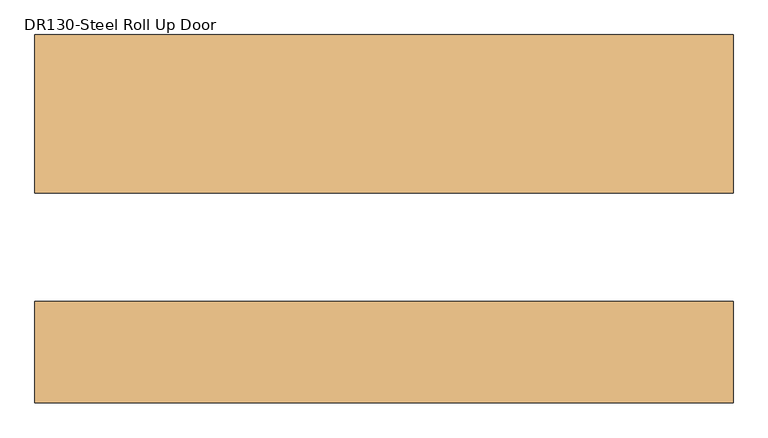
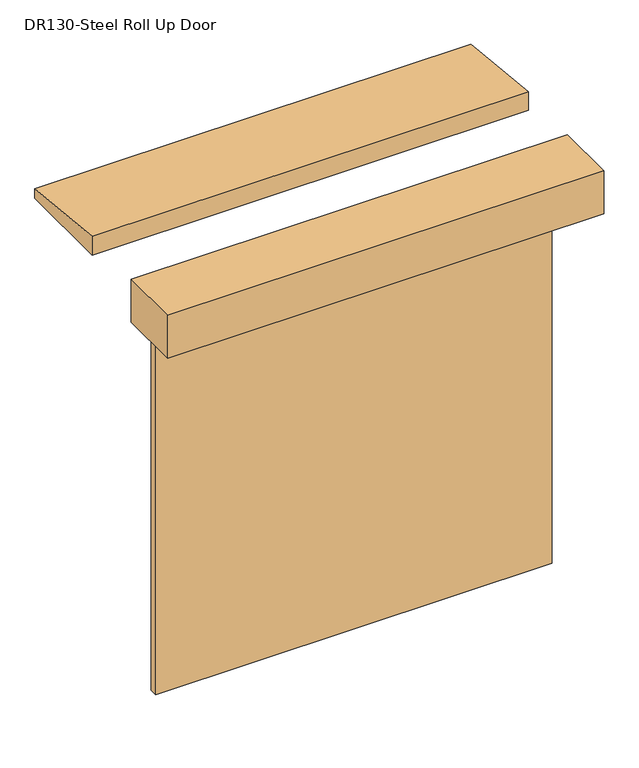
"""IFC4 building model written with IfcOpenShell, lengths in millimetres: door geometry, DR130-Steel Roll Up Door : DR131-Steel Roll Up Door-W4000xH4000mm."""

import ifcopenshell
import ifcopenshell.guid

model = None  # the IFC model being written
_history = None  # IfcOwnerHistory: only IFC2X3 demands one
_inside = {}  # id of a spatial element -> (the spatial element, [elements in it])
_under = {}  # id of a project, library or spatial element -> (it, [spatial elements below it])
_declared = {}  # id of a project -> (the project, [libraries it declares])
_typed = {}  # id of a type object -> (the type object, [elements of that type])
_made_of = {}  # id of a material, layer set ... -> (it, [elements and type objects made of it])


def new_model(schema):
    """Start an empty IFC model of exactly this schema.

    Asked for "IFC4X3", IfcOpenShell would pick the latest addendum, in which some entities
    have other attributes; the version numbers below select the first issue.
    IFC2X3 requires an IfcOwnerHistory on every rooted entity: one is made here for all.
    """
    global model, _history
    if schema == "IFC4X3":
        model = ifcopenshell.file(schema_version=(4, 3, 0, 0))
    else:
        model = ifcopenshell.file(schema=schema)
    _inside.clear()
    _under.clear()
    _declared.clear()
    _typed.clear()
    _made_of.clear()
    _history = None
    if model.schema == "IFC2X3":
        org = make("IfcOrganization", Name="unknown")
        user = make(
            "IfcPersonAndOrganization",
            ThePerson=make("IfcPerson", FamilyName="unknown"),
            TheOrganization=org,
        )
        app = make(
            "IfcApplication",
            ApplicationDeveloper=org,
            Version="unknown",
            ApplicationFullName="unknown",
            ApplicationIdentifier="unknown",
        )
        _history = make(
            "IfcOwnerHistory",
            OwningUser=user,
            OwningApplication=app,
            ChangeAction="ADDED",
            CreationDate=0,
        )
    return model


def make(cls, **values):
    """One entity of the class cls with the attributes given. An attribute that is None is left unset."""
    return model.create_entity(
        cls, **{name: value for name, value in values.items() if value is not None}
    )


def rooted(cls, **values):
    """An entity with a GlobalId (a new one), such as an element, a storey or a relation."""
    return make(cls, GlobalId=ifcopenshell.guid.new(), OwnerHistory=_history, **values)


def si_unit(unit_type, name, prefix=None):
    """IfcSIUnit, for example si_unit("LENGTHUNIT", "METRE", prefix="MILLI")."""
    return make("IfcSIUnit", UnitType=unit_type, Prefix=prefix, Name=name)


def assignment(units):
    """IfcUnitAssignment: the units of a project."""
    return None if units is None else make("IfcUnitAssignment", Units=units)


def point(xyz):
    """IfcCartesianPoint."""
    return None if xyz is None else make("IfcCartesianPoint", Coordinates=xyz)


def direction(xyz):
    """IfcDirection."""
    return None if xyz is None else make("IfcDirection", DirectionRatios=xyz)


def frame(location, z_axis=None, x_axis=None):
    """IfcAxis2Placement3D, a coordinate frame: its origin and axes. An axis left out is left unset."""
    return make(
        "IfcAxis2Placement3D",
        Location=point(location),
        Axis=direction(z_axis),
        RefDirection=direction(x_axis),
    )


def origin():
    """The frame at (0, 0, 0) with its axes left unset."""
    return frame((0.0, 0.0, 0.0))


def origin_with_axes():
    """The frame at (0, 0, 0) with the z axis (0, 0, 1) and the x axis (1, 0, 0) written out."""
    return frame((0.0, 0.0, 0.0), z_axis=(0.0, 0.0, 1.0), x_axis=(1.0, 0.0, 0.0))


def place(relative_to, where):
    """IfcLocalPlacement: puts the frame where relative to a parent placement (None: the world)."""
    return make(
        "IfcLocalPlacement", PlacementRelTo=relative_to, RelativePlacement=where
    )


def context(
    kind, dimensions, precision=None, world=None, true_north=None, identifier=None
):
    """IfcGeometricRepresentationContext, for example the 3D "Model" context."""
    return make(
        "IfcGeometricRepresentationContext",
        ContextIdentifier=identifier,
        ContextType=kind,
        CoordinateSpaceDimension=dimensions,
        Precision=precision,
        WorldCoordinateSystem=world,
        TrueNorth=true_north,
    )


def project(units=None, contexts=None):
    """IfcProject with its units and contexts."""
    return rooted(
        "IfcProject",
        Name="project",
        RepresentationContexts=contexts,
        UnitsInContext=assignment(units),
    )


def spatial(cls, under=None, at=None, **own):
    """A site, building, storey or space (cls), placed at a placement, below another one or the project."""
    s = rooted(cls, ObjectPlacement=at, **own)
    if under is not None:
        _under.setdefault(under.id(), (under, []))[1].append(s)
    return s


def polyline(points):
    """IfcPolyline through the points."""
    return make("IfcPolyline", Points=[point(p) for p in points])


def outline(outer, holes=None, kind="AREA"):
    """IfcArbitraryClosedProfileDef: a profile drawn as a closed curve; with holes, ...WithVoids."""
    if holes is None:
        return make("IfcArbitraryClosedProfileDef", ProfileType=kind, OuterCurve=outer)
    return make(
        "IfcArbitraryProfileDefWithVoids",
        ProfileType=kind,
        OuterCurve=outer,
        InnerCurves=holes,
    )


def extrude(swept, where, along, depth):
    """IfcExtrudedAreaSolid: the profile swept, set in the frame where, extruded along a direction by depth."""
    return make(
        "IfcExtrudedAreaSolid",
        SweptArea=swept,
        Position=where,
        ExtrudedDirection=direction(along),
        Depth=depth,
    )


def shape(context_of_items, identifier, shape_type, items):
    """IfcShapeRepresentation: the items that make up one representation, for example the "Body"."""
    return make(
        "IfcShapeRepresentation",
        ContextOfItems=context_of_items,
        RepresentationIdentifier=identifier,
        RepresentationType=shape_type,
        Items=items,
    )


def source(mapping_origin, context_of_items, identifier, shape_type, items):
    """IfcRepresentationMap: a shape defined once, which mapped items show again and again."""
    return make(
        "IfcRepresentationMap",
        MappingOrigin=mapping_origin,
        MappedRepresentation=shape(context_of_items, identifier, shape_type, items),
    )


def transform(
    local_origin,
    x_axis=None,
    y_axis=None,
    z_axis=None,
    scale=None,
    scale2=None,
    scale3=None,
    uniform=True,
):
    """IfcCartesianTransformationOperator3D, or its non-uniform kind. x_axis, y_axis, z_axis: its Axis1, 2, 3."""
    if uniform:
        return make(
            "IfcCartesianTransformationOperator3D",
            Axis1=direction(x_axis),
            Axis2=direction(y_axis),
            LocalOrigin=point(local_origin),
            Scale=scale,
            Axis3=direction(z_axis),
        )
    return make(
        "IfcCartesianTransformationOperator3DnonUniform",
        Axis1=direction(x_axis),
        Axis2=direction(y_axis),
        LocalOrigin=point(local_origin),
        Scale=scale,
        Axis3=direction(z_axis),
        Scale2=scale2,
        Scale3=scale3,
    )


def mapped(mapping_source, mapping_target):
    """IfcMappedItem: shows the shape of a source again, moved by a transform."""
    return make(
        "IfcMappedItem", MappingSource=mapping_source, MappingTarget=mapping_target
    )


def made_of(thing, what):
    """Note that an element or type object is made of a material, layer set ...; save() writes the relation."""
    if what is not None:
        _made_of.setdefault(what.id(), (what, []))[1].append(thing)
    return thing


def element(
    cls,
    number,
    at=None,
    inside=None,
    cuts=None,
    type_object=None,
    material=None,
    context=None,
    identifier="Body",
    shape_type=None,
    held_by="IfcProductDefinitionShape",
    body=None,
    shapes=None,
    **own,
):
    """One element of the class cls, such as IfcWall. Its Tag is "e" and its number.

    at: its placement. inside: the storey or other place that contains it. cuts: it is an
    opening in that element (IfcRelVoidsElement). A single representation is given by context,
    identifier, shape_type and body (its items); several are given by shapes. held_by: the class
    of the entity that holds the representations. save() writes the other relations.
    """
    e = rooted(cls, Tag="e%d" % number, ObjectPlacement=at, **own)
    if body is not None:
        shapes = [shape(context, identifier, shape_type, body)]
    if shapes is not None:
        e.Representation = make(held_by, Representations=shapes)
    if inside is not None:
        _inside.setdefault(inside.id(), (inside, []))[1].append(e)
    if cuts is not None:
        rooted(
            "IfcRelVoidsElement", RelatingBuildingElement=cuts, RelatedOpeningElement=e
        )
    if type_object is not None:
        _typed.setdefault(type_object.id(), (type_object, []))[1].append(e)
    return made_of(e, material)


def aggregate(whole, parts):
    """IfcRelAggregates: a whole, such as a stair, and the parts it consists of."""
    return rooted("IfcRelAggregates", RelatingObject=whole, RelatedObjects=parts)


def save(model, path):
    """Write the relations noted so far, then the file.

    IfcRelAggregates (storeys below a building ...), IfcRelContainedInSpatialStructure (elements
    in a storey), IfcRelDefinesByType, IfcRelAssociatesMaterial and IfcRelDeclares: one each for
    every whole, place, type object, material and project.
    """
    for whole, parts in _under.values():
        aggregate(whole, parts)
    for where, things in _inside.values():
        rooted(
            "IfcRelContainedInSpatialStructure",
            RelatedElements=things,
            RelatingStructure=where,
        )
    for kind, things in _typed.values():
        rooted("IfcRelDefinesByType", RelatedObjects=things, RelatingType=kind)
    for what, things in _made_of.values():
        rooted("IfcRelAssociatesMaterial", RelatedObjects=things, RelatingMaterial=what)
    for by, libraries in _declared.values():
        rooted("IfcRelDeclares", RelatingContext=by, RelatedDefinitions=libraries)
    model.write(path)


def dr130_steel_roll_up_door_abb043e2(model_context):
    return source(origin(), model_context, "Body", "SweptSolid", [
        extrude(outline(polyline([(1175.0, 4300.0), (175.0, 4300.0), (175.0, 4500.0), (1175.0, 4400.0), (1175.0, 4300.0)])), frame((-2203.2, 0.0, 0.0), z_axis=(1.0, 0.0, 0.0), x_axis=(0.0, 1.0, 0.0)), (0.0, 0.0, 1.0), 4406.4),
        extrude(outline(polyline([(2203.2, -1148.8), (-2203.2, -1148.8), (-2203.2, -510.0), (2203.2, -510.0), (2203.2, -1148.8)])), frame((0.0, 0.0, 4000.0), z_axis=(0.0, 0.0, 1.0), x_axis=(1.0, 0.0, 0.0)), (0.0, 0.0, 1.0), 457.2),
        extrude(outline(polyline([(2000.0, -510.0), (2000.0, -590.0), (-2000.0, -590.0), (-2000.0, -510.0), (2000.0, -510.0)])), origin_with_axes(), (0.0, 0.0, 1.0), 4000.0),
    ])


if __name__ == "__main__":
    model = new_model("IFC4")
    model_context = context("Model", 3, world=origin())
    ifc_project = project(units=[si_unit("LENGTHUNIT", "METRE", prefix="MILLI")], contexts=[model_context])
    site = spatial("IfcSite", under=ifc_project)
    building = spatial("IfcBuilding", under=site)
    placement = place(None, origin())
    dr130_steel_roll_up_door_shape = dr130_steel_roll_up_door_abb043e2(model_context)
    element("IfcDoor", 1, ObjectType="DR130-Steel Roll Up Door : DR131-Steel Roll Up Door-W4000xH4000mm", at=placement, inside=building, context=model_context, shape_type="MappedRepresentation", body=[
        mapped(dr130_steel_roll_up_door_shape, transform((0.0, 0.0, 0.0), x_axis=(1.0, 0.0, 0.0), y_axis=(0.0, 1.0, 0.0), z_axis=(0.0, 0.0, 1.0))),
    ])
    save(model, "model.ifc")

# Revit data of these elements
# Type "DR130-Steel Roll Up Door : DR131-Steel Roll Up Door-W4000xH4000mm"
#   Type Mark = "361"
#   Construction Type Id = "MDOOR"
#   Assembly Code = "B2030400"
#   Analytic Construction = "<None>"
#   Thickness = 80 mm
#   Thermal Resistance (R) = 0.270117 (m²·K)/W
#   Rough Width [instance default] = 4000 mm
#   Rough Height [instance default] = 4000 mm
#   Offset [instance default] = 1000 mm
#   Heat Transfer Coefficient (U) = 3.7021 W/(m²·K)
#   Height [instance default] = 4000 mm
#   Width [instance default] = 4000 mm
#   Function = 1
#   Define Thermal Properties by = 1
#   Canopy [instance default] = yes
#   Roller Material = A04AQ112-00002_Steel Roll Up Door
#   Roller Box Material = A04AQ112-00002_Steel Roll Up Door
#   Visual Light Transmittance = 0
#   Solar Heat Gain Coefficient = 0
#   Wall Closure = (empty or 0)
# Element 1 (IfcDoor, "DR130-Steel Roll Up Door : DR131-Steel Roll Up Door-W4000xH4000mm")
#   Offset = 550 mm
#   Materials on its faces: "A04AQ112-00002_Steel Roll Up Door"
# Materials
#   "A04AQ112-00002_Steel Roll Up Door": class "금속", colour RGB 247 247 247, transparency 0, Description = "Steel Door", W00) Work Master Code = "A04AQ112-00002", W01) Work Master_Lv1 = "Finishing Work", W02) Work Master_Lv2 = "Door & Window Work", W03) Work Master_Spec.1 = "Steel Roll Up Door w/ Steel Frame", W04) Work Master_Spec.2 = "Fire Protective Rating: N/A, Motorized Type", W05) Work Master_Spec.3 = "w/ Hardware & Accessories", Cost = 0
